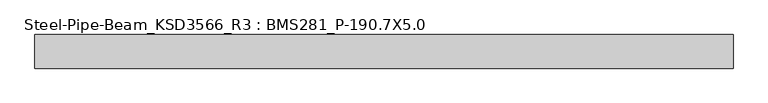
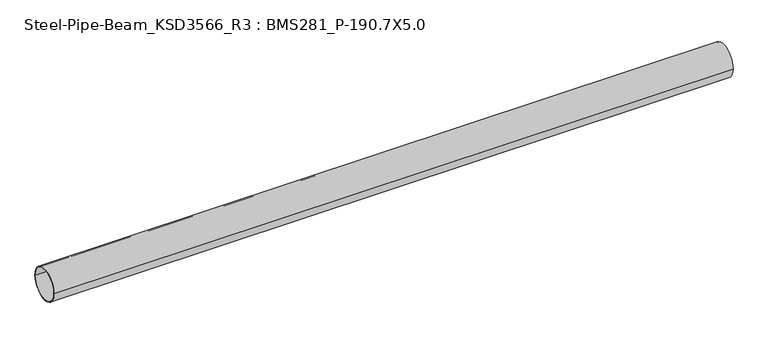
"""IFC4 building model written with IfcOpenShell, lengths in millimetres: member geometry, Steel-Pipe-Beam_KSD3566_R3 : BMS281_P-190.7X5.0."""

from ifc_helpers import new_model, si_unit, point, frame, origin, origin_2d, place, context, project, spatial, circle_curve, trimmed, segment, composite_curve, outline, extrude, source, transform, mapped, element, save


def steel_pipe_beam_ksd3566_r3_bms281_p_190_7x5_0_4dc1edcf(model_context):
    return source(origin(), model_context, "Body", "SweptSolid", [
        extrude(outline(composite_curve([segment(trimmed(circle_curve(origin_2d(), 95.35), [point((-95.35, 0.0))], [point((95.35, 0.0))], False, "CARTESIAN"), True, "CONTINUOUS"), segment(trimmed(circle_curve(origin_2d(), 95.35), [point((95.35, 0.0))], [point((-95.35, 0.0))], False, "CARTESIAN"), True, "CONTINUOUS")], self_intersect=False), holes=[composite_curve([segment(trimmed(circle_curve(origin_2d(), 90.35), [point((90.35, 0.0))], [point((-90.35, 0.0))], True, "CARTESIAN"), True, "CONTINUOUS"), segment(trimmed(circle_curve(origin_2d(), 90.35), [point((-90.35, 0.0))], [point((90.35, 0.0))], True, "CARTESIAN"), True, "CONTINUOUS")], self_intersect=False)]), frame((-1965.4784034, 0.0, 0.0), z_axis=(1.0, 0.0, 0.0), x_axis=(0.0, 1.0, 0.0)), (0.0, 0.0, 1.0), 3954.0532033),
    ])


if __name__ == "__main__":
    model = new_model("IFC4")
    model_context = context("Model", 3, world=origin())
    ifc_project = project(units=[si_unit("LENGTHUNIT", "METRE", prefix="MILLI")], contexts=[model_context])
    site = spatial("IfcSite", under=ifc_project)
    building = spatial("IfcBuilding", under=site)
    placement = place(None, origin())
    steel_pipe_beam_ksd3566_r3_bms281_p_190_7x5_0_shape = steel_pipe_beam_ksd3566_r3_bms281_p_190_7x5_0_4dc1edcf(model_context)
    element("IfcMember", 1, ObjectType="Steel-Pipe-Beam_KSD3566_R3 : BMS281_P-190.7X5.0", at=placement, inside=building, context=model_context, shape_type="MappedRepresentation", body=[
        mapped(steel_pipe_beam_ksd3566_r3_bms281_p_190_7x5_0_shape, transform((0.0, 0.0, 0.0), x_axis=(1.0, 0.0, 0.0), y_axis=(0.0, 1.0, 0.0), z_axis=(0.0, 0.0, 1.0))),
    ])
    save(model, "model.ifc")

# Revit data of these elements
# Type "Steel-Pipe-Beam_KSD3566_R3 : BMS281_P-190.7X5.0"
#   Keynote = "P-190.7X5.0"
#   SteelWeight = "Light"
#   t = 0.0050 m
#   Surface Area = 0.599102 m²/m
#   Section Area = 29.1697 cm²
#   Mass per Unit Length = 22.8982 kg/m
#   Length [instance default] = 1.5000 m
#   D = 0.1907 m
#   hec_material4 [instance default] = none
#   hec_material3 [instance default] = none
#   hec_material2 [instance default] = none
#   hec_material1 [instance default] = none
#   Structural Material [instance default] = Steel, 45-345
#   Assembly Code = ""
# Element 1 (IfcMember, "Steel-Pipe-Beam_KSD3566_R3 : BMS281_P-190.7X5.0")
#   Structural Material = none
# Materials
#   "Steel, 45-345": class "Metal", colour RGB 189 187 185, transparency 0, Description = "Steel 345 MPa", Cost = 0
